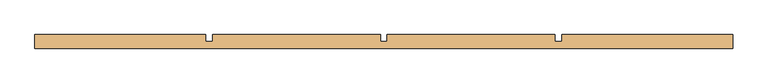
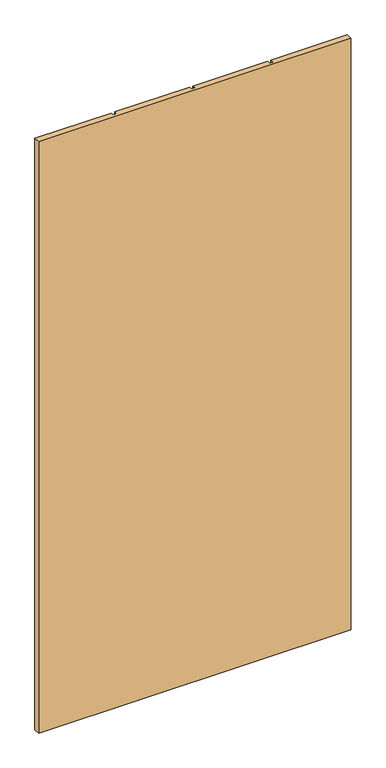
"""IFC4 building model written with IfcOpenShell, lengths in millimetres: door geometry, BA_Bi-fold door : AD_Bi-fold door - 100cm."""

from ifc_helpers import new_model, si_unit, origin, origin_with_axes, place, context, project, spatial, polyline, outline, extrude, source, transform, mapped, element, save


def door_88445510(model_context):
    return source(origin(), model_context, "Body", "SweptSolid", [
        extrude(outline(polyline([(255.0, 10.0), (500.0, 10.0), (500.0, -10.0), (-500.0, -10.0), (-500.0, 10.0), (-255.0, 10.0), (-255.0, 0.0), (-245.0, 0.0), (-245.0, 10.0), (-5.0, 10.0), (-5.0, 0.0), (5.0, 0.0), (5.0, 10.0), (245.0, 10.0), (245.0, 0.0), (255.0, 0.0), (255.0, 10.0)])), origin_with_axes(), (0.0, 0.0, 1.0), 2000.0),
    ])


if __name__ == "__main__":
    model = new_model("IFC4")
    model_context = context("Model", 3, world=origin())
    ifc_project = project(units=[si_unit("LENGTHUNIT", "METRE", prefix="MILLI")], contexts=[model_context])
    site = spatial("IfcSite", under=ifc_project)
    building = spatial("IfcBuilding", under=site)
    placement = place(None, origin())
    door_shape = door_88445510(model_context)
    element("IfcDoor", 1, ObjectType="BA_Bi-fold door : AD_Bi-fold door - 100cm", at=placement, inside=building, context=model_context, shape_type="MappedRepresentation", body=[
        mapped(door_shape, transform((0.0, 0.0, 0.0), x_axis=(1.0, 0.0, 0.0), y_axis=(0.0, 1.0, 0.0), z_axis=(0.0, 0.0, 1.0))),
    ])
    save(model, "model.ifc")

# Revit data of these elements
# Type "BA_Bi-fold door : AD_Bi-fold door - 100cm"
#   Type Mark = "45"
#   Frame Projection Ext. = 25 mm
#   Frame Projection Int. = 25 mm
#   Frame Width = 75 mm
#   Height = 2000 mm
#   Width = 1000 mm
#   Define Thermal Properties by = 1
#   160cm = no
#   140cm = no
#   120cm = no
#   100cm = yes
#   Function = (empty or 0)
#   Wall Closure = (empty or 0)
# Element 1 (IfcDoor, "BA_Bi-fold door : AD_Bi-fold door - 100cm")
#   Materials on its faces: "Default"
# Materials
#   "Default": class "Generic", colour RGB 255 255 255, transparency 0, Cost = 0
